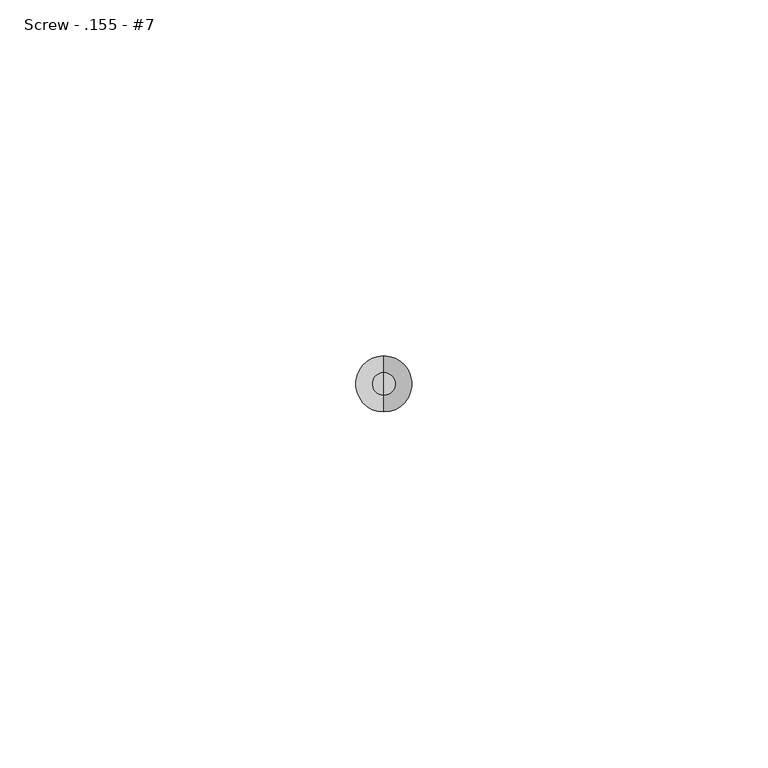
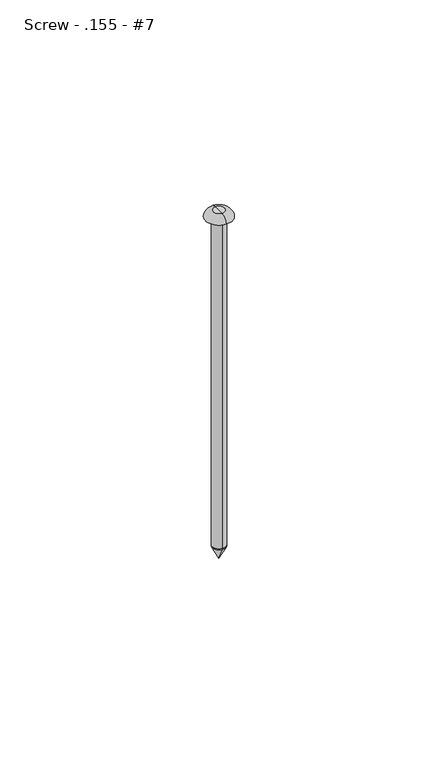
"""IFC4 building model written with IfcOpenShell, lengths in millimetres: fastener geometry, 060523 - W_P_C - Fastenings - Generic : Screw - .155 - #7."""

from ifc_helpers import new_model, si_unit, point, frame, origin, origin_2d, place, context, project, spatial, polyline, circle_curve, ellipse_curve, trimmed, segment, composite_curve, outline, extrude, source, transform, mapped, element, save
from ifc_brep_helpers import plane_surface, revolved_surface, advanced_brep


def screw_155_7_76f66364(model_context):
    return source(origin(), model_context, "Body", "SolidModel", [
        advanced_brep(
        [(0.0, -1.9685, -101.6), (0.0, 1.9685, -101.6), (0.0, 0.0, -101.6), (0.0, 0.0, -105.537)],
        [
            (0, 1, circle_curve(frame((0.0, 0.0, -101.6), z_axis=(0.0, 0.0, 1.0), x_axis=(0.0, 1.0, 0.0)), 1.9685)),
            (1, 2),
            (2, 0),
            (1, 0, circle_curve(frame((0.0, 0.0, -101.6), z_axis=(0.0, 0.0, 1.0), x_axis=(0.0, 1.0, 0.0)), 1.9685)),
            (3, 1),
            (0, 3),
        ],
        [
            plane_surface(frame((0.0, 0.0, -101.6), z_axis=(0.0, 0.0, 1.0), x_axis=(0.0, 1.0, 0.0))),
            revolved_surface(polyline([(0.0, 1.9685, -101.6), (0.0, 0.0, -105.537)]), (0.0, 0.0, -103.0840259), (0.0, 0.0, -1.0)),
        ],
        [
            (0, [[1, 2, 3]]),
            (0, [[4, -3, -2]]),
            (1, [[5, -1, 6]]),
            (1, [[-6, -4, -5]]),
        ],
    ),
        advanced_brep(
        [(0.0, 3.937, 0.0), (0.0, -3.937, 0.0), (0.0, 0.0, 0.0), (0.0, 0.0, 1.9685), (0.0, -1.5875, 1.9685), (0.0, 1.5875, 1.9685)],
        [
            (0, 1, circle_curve(frame((0.0, 0.0, 0.0), z_axis=(0.0, 0.0, -1.0), x_axis=(0.0, -1.0, 0.0)), 3.937)),
            (1, 2),
            (2, 0),
            (1, 0, circle_curve(frame((0.0, 0.0, 0.0), z_axis=(0.0, 0.0, -1.0), x_axis=(0.0, -1.0, 0.0)), 3.937)),
            (3, 4),
            (4, 5, circle_curve(frame((0.0, 0.0, 1.9685), z_axis=(0.0, 0.0, 1.0), x_axis=(0.0, -1.0, 0.0)), 1.5875)),
            (5, 3),
            (5, 4, circle_curve(frame((0.0, 0.0, 1.9685), z_axis=(0.0, 0.0, 1.0), x_axis=(0.0, -1.0, 0.0)), 1.5875)),
            (4, 1, circle_curve(frame((0.0, -1.5875, -0.417871), z_axis=(1.0, 0.0, 0.0), x_axis=(0.0, -1.0, 0.0)), 2.386371)),
            (0, 5, circle_curve(frame((0.0, 1.5875, -0.417871), z_axis=(1.0, 0.0, 0.0), x_axis=(0.0, 1.0, 0.0)), 2.386371)),
        ],
        [
            plane_surface(frame((0.0, 0.0, 0.0), z_axis=(0.0, 0.0, -1.0), x_axis=(0.0, -1.0, 0.0))),
            plane_surface(frame((0.0, 0.0, 1.9685), z_axis=(0.0, 0.0, 1.0), x_axis=(0.0, -1.0, 0.0))),
            revolved_surface(trimmed(ellipse_curve(frame((0.0, -1.5875, -0.417871), z_axis=(-1.0, 0.0, 0.0), x_axis=(0.0, -1.0, 0.0)), 2.386371, 2.386371), [point((0.0, -3.937, 0.0))], [point((0.0, -1.5875, 1.9685))], True, "CARTESIAN"), (0.0, 0.0, 1.4840259), (0.0, 0.0, 1.0)),
        ],
        [
            (0, [[1, 2, 3]]),
            (0, [[4, -3, -2]]),
            (1, [[5, 6, 7]]),
            (1, [[-7, 8, -5]]),
            (2, [[-6, 9, -1, 10]]),
            (2, [[-8, -10, -4, -9]]),
        ],
    ),
        extrude(outline(composite_curve([segment(trimmed(circle_curve(origin_2d(), 1.9685), [point((0.0, -1.9685))], [point((0.0, 1.9685))], False, "CARTESIAN"), True, "CONTINUOUS"), segment(trimmed(circle_curve(origin_2d(), 1.9685), [point((0.0, 1.9685))], [point((0.0, -1.9685))], False, "CARTESIAN"), True, "CONTINUOUS")], self_intersect=False)), frame((0.0, 0.0, -101.6), z_axis=(0.0, 0.0, 1.0), x_axis=(1.0, 0.0, 0.0)), (0.0, 0.0, 1.0), 101.6),
    ])


if __name__ == "__main__":
    model = new_model("IFC4")
    model_context = context("Model", 3, world=origin())
    ifc_project = project(units=[si_unit("LENGTHUNIT", "METRE", prefix="MILLI")], contexts=[model_context])
    site = spatial("IfcSite", under=ifc_project)
    building = spatial("IfcBuilding", under=site)
    placement = place(None, origin())
    screw_155_7_shape = screw_155_7_76f66364(model_context)
    element("IfcFastener", 1, ObjectType="060523 - W_P_C - Fastenings - Generic : Screw - .155 - #7", at=placement, inside=building, context=model_context, shape_type="MappedRepresentation", body=[
        mapped(screw_155_7_shape, transform((0.0, 0.0, 0.0), x_axis=(1.0, 0.0, 0.0), y_axis=(0.0, 1.0, 0.0), z_axis=(0.0, 0.0, 1.0))),
    ])
    save(model, "model.ifc")

# Revit data of these elements
# Type "060523 - W_P_C - Fastenings - Generic : Screw - .155 - #7"
#   Washer_Thickness = 0' - 0.00333"
#   Washer Radius = 0' - 0.0875"
#   Washer Offset - Head = 0' - 0"
#   Washer Offset = 0' - 0"
#   Thickness_of_Substrate [instance default] = 0' - 1"
#   Side = 0' - 0 37/64"
#   Radius = 0' - 0.0775"
#   Length [instance default] = 0' - 4"
#   Head Size = 0' - 1"
#   Head Radius = 0' - 0 1/2"
#   Head Height = 0' - 0.01"
#   Double Diameter = 0' - 0.31"
#   Diameter = 0' - 0.155"
#   Default Elevation = 4' - 0"
#   Washer_Nut_Visibility = no
#   Washer_Head_Visibility = no
#   Round_Head_Visibility = yes
#   Point Visibility = yes
#   Nut_Visibility = no
#   Hex_Head_Visiblilty = no
#   Washer Material = none
#   Bolt Material (Size) = AT SILL - FASTENER AT 24" O.C.
# Element 1 (IfcFastener, "060523 - W_P_C - Fastenings - Generic : Screw - .155 - #7")
#   Materials on its faces: "AT SILL - FASTENER AT 24\" O.C."
# Materials
#   "AT SILL - FASTENER AT 24\" O.C.": class "Generic", colour RGB 120 120 120, transparency 0, Cost = 0
